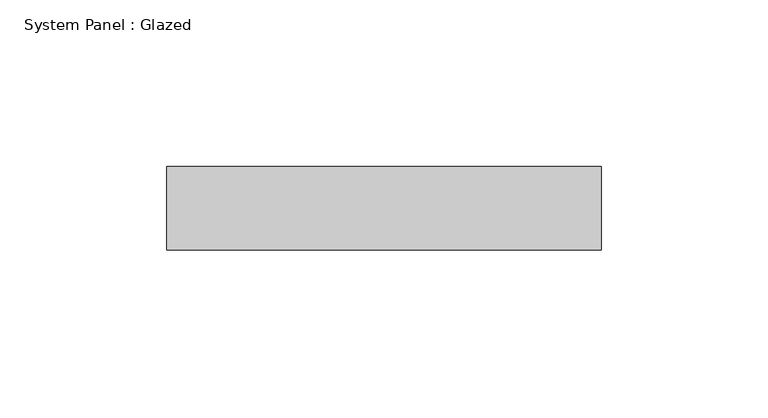
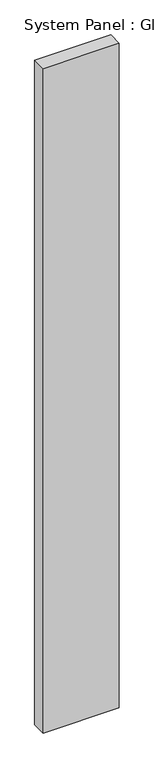
"""IFC4 building model written with IfcOpenShell, lengths in millimetres: plate geometry, System Panel : Glazed."""

from ifc_helpers import new_model, si_unit, origin, origin_with_axes, place, context, project, spatial, polyline, outline, extrude, source, transform, mapped, element, save


def system_panel_glazed_aaeb877f(model_context):
    return source(origin(), model_context, "Body", "SweptSolid", [
        extrude(outline(polyline([(65.0, 24.5), (-65.0, 24.5), (-65.0, 49.5), (65.0, 49.5), (65.0, 24.5)])), origin_with_axes(), (0.0, 0.0, 1.0), 1200.0),
    ])


if __name__ == "__main__":
    model = new_model("IFC4")
    model_context = context("Model", 3, world=origin())
    ifc_project = project(units=[si_unit("LENGTHUNIT", "METRE", prefix="MILLI")], contexts=[model_context])
    site = spatial("IfcSite", under=ifc_project)
    building = spatial("IfcBuilding", under=site)
    placement = place(None, origin())
    system_panel_glazed_shape = system_panel_glazed_aaeb877f(model_context)
    element("IfcPlate", 1, ObjectType="System Panel : Glazed", at=placement, inside=building, context=model_context, shape_type="MappedRepresentation", body=[
        mapped(system_panel_glazed_shape, transform((0.0, 0.0, 0.0), x_axis=(1.0, 0.0, 0.0), y_axis=(0.0, 1.0, 0.0), z_axis=(0.0, 0.0, 1.0))),
    ])
    save(model, "model.ifc")

# Revit data of these elements
# Element 1 (IfcPlate, "System Panel : Glazed")
#   Materials on its faces: "Glass"
# Materials
#   "Glass": class "Glass", colour RGB 218 227 224, transparency 0.85, Description = "Soda Lime Glass", Cost = 0
